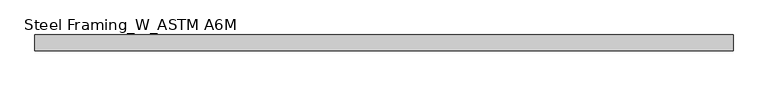
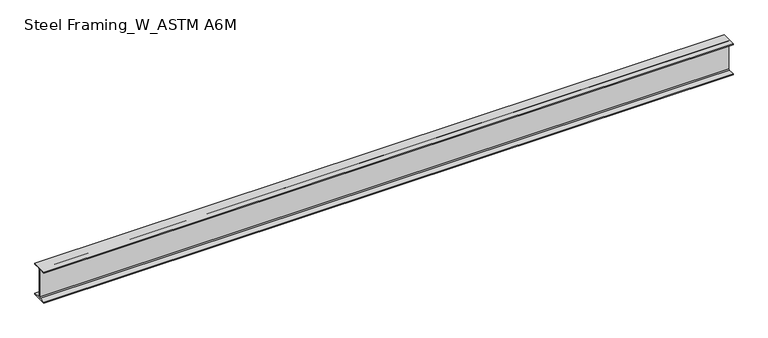
"""IFC4 building model written with IfcOpenShell, lengths in millimetres: beam geometry, Steel Framing_W_ASTM A6M : H_SB_AR_S02_W360x51_G3."""

import ifcopenshell
import ifcopenshell.guid

model = None  # the IFC model being written
_history = None  # IfcOwnerHistory: only IFC2X3 demands one
_inside = {}  # id of a spatial element -> (the spatial element, [elements in it])
_under = {}  # id of a project, library or spatial element -> (it, [spatial elements below it])
_declared = {}  # id of a project -> (the project, [libraries it declares])
_typed = {}  # id of a type object -> (the type object, [elements of that type])
_made_of = {}  # id of a material, layer set ... -> (it, [elements and type objects made of it])


def new_model(schema):
    """Start an empty IFC model of exactly this schema.

    Asked for "IFC4X3", IfcOpenShell would pick the latest addendum, in which some entities
    have other attributes; the version numbers below select the first issue.
    IFC2X3 requires an IfcOwnerHistory on every rooted entity: one is made here for all.
    """
    global model, _history
    if schema == "IFC4X3":
        model = ifcopenshell.file(schema_version=(4, 3, 0, 0))
    else:
        model = ifcopenshell.file(schema=schema)
    _inside.clear()
    _under.clear()
    _declared.clear()
    _typed.clear()
    _made_of.clear()
    _history = None
    if model.schema == "IFC2X3":
        org = make("IfcOrganization", Name="unknown")
        user = make(
            "IfcPersonAndOrganization",
            ThePerson=make("IfcPerson", FamilyName="unknown"),
            TheOrganization=org,
        )
        app = make(
            "IfcApplication",
            ApplicationDeveloper=org,
            Version="unknown",
            ApplicationFullName="unknown",
            ApplicationIdentifier="unknown",
        )
        _history = make(
            "IfcOwnerHistory",
            OwningUser=user,
            OwningApplication=app,
            ChangeAction="ADDED",
            CreationDate=0,
        )
    return model


def make(cls, **values):
    """One entity of the class cls with the attributes given. An attribute that is None is left unset."""
    return model.create_entity(
        cls, **{name: value for name, value in values.items() if value is not None}
    )


def rooted(cls, **values):
    """An entity with a GlobalId (a new one), such as an element, a storey or a relation."""
    return make(cls, GlobalId=ifcopenshell.guid.new(), OwnerHistory=_history, **values)


def si_unit(unit_type, name, prefix=None):
    """IfcSIUnit, for example si_unit("LENGTHUNIT", "METRE", prefix="MILLI")."""
    return make("IfcSIUnit", UnitType=unit_type, Prefix=prefix, Name=name)


def assignment(units):
    """IfcUnitAssignment: the units of a project."""
    return None if units is None else make("IfcUnitAssignment", Units=units)


def point(xyz):
    """IfcCartesianPoint."""
    return None if xyz is None else make("IfcCartesianPoint", Coordinates=xyz)


def direction(xyz):
    """IfcDirection."""
    return None if xyz is None else make("IfcDirection", DirectionRatios=xyz)


def frame(location, z_axis=None, x_axis=None):
    """IfcAxis2Placement3D, a coordinate frame: its origin and axes. An axis left out is left unset."""
    return make(
        "IfcAxis2Placement3D",
        Location=point(location),
        Axis=direction(z_axis),
        RefDirection=direction(x_axis),
    )


def frame_2d(location, x_axis=None):
    """IfcAxis2Placement2D, a coordinate frame in the plane: its origin and x axis."""
    return make(
        "IfcAxis2Placement2D", Location=point(location), RefDirection=direction(x_axis)
    )


def origin():
    """The frame at (0, 0, 0) with its axes left unset."""
    return frame((0.0, 0.0, 0.0))


def place(relative_to, where):
    """IfcLocalPlacement: puts the frame where relative to a parent placement (None: the world)."""
    return make(
        "IfcLocalPlacement", PlacementRelTo=relative_to, RelativePlacement=where
    )


def context(
    kind, dimensions, precision=None, world=None, true_north=None, identifier=None
):
    """IfcGeometricRepresentationContext, for example the 3D "Model" context."""
    return make(
        "IfcGeometricRepresentationContext",
        ContextIdentifier=identifier,
        ContextType=kind,
        CoordinateSpaceDimension=dimensions,
        Precision=precision,
        WorldCoordinateSystem=world,
        TrueNorth=true_north,
    )


def project(units=None, contexts=None):
    """IfcProject with its units and contexts."""
    return rooted(
        "IfcProject",
        Name="project",
        RepresentationContexts=contexts,
        UnitsInContext=assignment(units),
    )


def spatial(cls, under=None, at=None, **own):
    """A site, building, storey or space (cls), placed at a placement, below another one or the project."""
    s = rooted(cls, ObjectPlacement=at, **own)
    if under is not None:
        _under.setdefault(under.id(), (under, []))[1].append(s)
    return s


def polyline(points):
    """IfcPolyline through the points."""
    return make("IfcPolyline", Points=[point(p) for p in points])


def circle_curve(where, radius):
    """IfcCircle in the frame where."""
    return make("IfcCircle", Position=where, Radius=radius)


def trimmed(basis, trim1, trim2, sense, master):
    """IfcTrimmedCurve: the piece of a basis curve between two trims."""
    return make(
        "IfcTrimmedCurve",
        BasisCurve=basis,
        Trim1=trim1,
        Trim2=trim2,
        SenseAgreement=sense,
        MasterRepresentation=master,
    )


def segment(curve, same_sense, transition):
    """IfcCompositeCurveSegment."""
    return make(
        "IfcCompositeCurveSegment",
        Transition=transition,
        SameSense=same_sense,
        ParentCurve=curve,
    )


def composite_curve(segments, self_intersect=None):
    """IfcCompositeCurve: segments joined end to end."""
    return make("IfcCompositeCurve", Segments=segments, SelfIntersect=self_intersect)


def outline(outer, holes=None, kind="AREA"):
    """IfcArbitraryClosedProfileDef: a profile drawn as a closed curve; with holes, ...WithVoids."""
    if holes is None:
        return make("IfcArbitraryClosedProfileDef", ProfileType=kind, OuterCurve=outer)
    return make(
        "IfcArbitraryProfileDefWithVoids",
        ProfileType=kind,
        OuterCurve=outer,
        InnerCurves=holes,
    )


def extrude(swept, where, along, depth):
    """IfcExtrudedAreaSolid: the profile swept, set in the frame where, extruded along a direction by depth."""
    return make(
        "IfcExtrudedAreaSolid",
        SweptArea=swept,
        Position=where,
        ExtrudedDirection=direction(along),
        Depth=depth,
    )


def shape(context_of_items, identifier, shape_type, items):
    """IfcShapeRepresentation: the items that make up one representation, for example the "Body"."""
    return make(
        "IfcShapeRepresentation",
        ContextOfItems=context_of_items,
        RepresentationIdentifier=identifier,
        RepresentationType=shape_type,
        Items=items,
    )


def source(mapping_origin, context_of_items, identifier, shape_type, items):
    """IfcRepresentationMap: a shape defined once, which mapped items show again and again."""
    return make(
        "IfcRepresentationMap",
        MappingOrigin=mapping_origin,
        MappedRepresentation=shape(context_of_items, identifier, shape_type, items),
    )


def transform(
    local_origin,
    x_axis=None,
    y_axis=None,
    z_axis=None,
    scale=None,
    scale2=None,
    scale3=None,
    uniform=True,
):
    """IfcCartesianTransformationOperator3D, or its non-uniform kind. x_axis, y_axis, z_axis: its Axis1, 2, 3."""
    if uniform:
        return make(
            "IfcCartesianTransformationOperator3D",
            Axis1=direction(x_axis),
            Axis2=direction(y_axis),
            LocalOrigin=point(local_origin),
            Scale=scale,
            Axis3=direction(z_axis),
        )
    return make(
        "IfcCartesianTransformationOperator3DnonUniform",
        Axis1=direction(x_axis),
        Axis2=direction(y_axis),
        LocalOrigin=point(local_origin),
        Scale=scale,
        Axis3=direction(z_axis),
        Scale2=scale2,
        Scale3=scale3,
    )


def mapped(mapping_source, mapping_target):
    """IfcMappedItem: shows the shape of a source again, moved by a transform."""
    return make(
        "IfcMappedItem", MappingSource=mapping_source, MappingTarget=mapping_target
    )


def made_of(thing, what):
    """Note that an element or type object is made of a material, layer set ...; save() writes the relation."""
    if what is not None:
        _made_of.setdefault(what.id(), (what, []))[1].append(thing)
    return thing


def element(
    cls,
    number,
    at=None,
    inside=None,
    cuts=None,
    type_object=None,
    material=None,
    context=None,
    identifier="Body",
    shape_type=None,
    held_by="IfcProductDefinitionShape",
    body=None,
    shapes=None,
    **own,
):
    """One element of the class cls, such as IfcWall. Its Tag is "e" and its number.

    at: its placement. inside: the storey or other place that contains it. cuts: it is an
    opening in that element (IfcRelVoidsElement). A single representation is given by context,
    identifier, shape_type and body (its items); several are given by shapes. held_by: the class
    of the entity that holds the representations. save() writes the other relations.
    """
    e = rooted(cls, Tag="e%d" % number, ObjectPlacement=at, **own)
    if body is not None:
        shapes = [shape(context, identifier, shape_type, body)]
    if shapes is not None:
        e.Representation = make(held_by, Representations=shapes)
    if inside is not None:
        _inside.setdefault(inside.id(), (inside, []))[1].append(e)
    if cuts is not None:
        rooted(
            "IfcRelVoidsElement", RelatingBuildingElement=cuts, RelatedOpeningElement=e
        )
    if type_object is not None:
        _typed.setdefault(type_object.id(), (type_object, []))[1].append(e)
    return made_of(e, material)


def aggregate(whole, parts):
    """IfcRelAggregates: a whole, such as a stair, and the parts it consists of."""
    return rooted("IfcRelAggregates", RelatingObject=whole, RelatedObjects=parts)


def save(model, path):
    """Write the relations noted so far, then the file.

    IfcRelAggregates (storeys below a building ...), IfcRelContainedInSpatialStructure (elements
    in a storey), IfcRelDefinesByType, IfcRelAssociatesMaterial and IfcRelDeclares: one each for
    every whole, place, type object, material and project.
    """
    for whole, parts in _under.values():
        aggregate(whole, parts)
    for where, things in _inside.values():
        rooted(
            "IfcRelContainedInSpatialStructure",
            RelatedElements=things,
            RelatingStructure=where,
        )
    for kind, things in _typed.values():
        rooted("IfcRelDefinesByType", RelatedObjects=things, RelatingType=kind)
    for what, things in _made_of.values():
        rooted("IfcRelAssociatesMaterial", RelatedObjects=things, RelatingMaterial=what)
    for by, libraries in _declared.values():
        rooted("IfcRelDeclares", RelatingContext=by, RelatedDefinitions=libraries)
    model.write(path)


def steel_framing_w_astm_a6m_5f06bcad(model_context):
    return source(origin(), model_context, "Body", "SweptSolid", [
        extrude(outline(composite_curve([segment(polyline([(85.5, -166.4), (85.5, -178.0), (-85.5, -178.0), (-85.5, -166.4), (-13.72, -166.4)]), True, "CONTINUOUS"), segment(trimmed(circle_curve(frame_2d((-13.72, -156.3)), 10.1), [point((-13.72, -166.4))], [point((-3.62, -156.3))], True, "CARTESIAN"), True, "CONTINUOUS"), segment(polyline([(-3.62, -156.3), (-3.62, 156.3)]), True, "CONTINUOUS"), segment(trimmed(circle_curve(frame_2d((-13.72, 156.3)), 10.1), [point((-3.62, 156.3))], [point((-13.72, 166.4))], True, "CARTESIAN"), True, "CONTINUOUS"), segment(polyline([(-13.72, 166.4), (-85.5, 166.4), (-85.5, 178.0), (85.5, 178.0), (85.5, 166.4), (13.72, 166.4)]), True, "CONTINUOUS"), segment(trimmed(circle_curve(frame_2d((13.72, 156.3)), 10.1), [point((13.72, 166.4))], [point((3.62, 156.3))], True, "CARTESIAN"), True, "CONTINUOUS"), segment(polyline([(3.62, 156.3), (3.62, -156.3)]), True, "CONTINUOUS"), segment(trimmed(circle_curve(frame_2d((13.72, -156.3)), 10.1), [point((3.62, -156.3))], [point((13.72, -166.4))], True, "CARTESIAN"), True, "CONTINUOUS"), segment(polyline([(13.72, -166.4), (85.5, -166.4)]), True, "CONTINUOUS")], self_intersect=False)), frame((-3753.8, 0.0, 0.0), z_axis=(1.0, 0.0, 0.0), x_axis=(0.0, 1.0, 0.0)), (0.0, 0.0, 1.0), 7507.6),
    ])


if __name__ == "__main__":
    model = new_model("IFC4")
    model_context = context("Model", 3, world=origin())
    ifc_project = project(units=[si_unit("LENGTHUNIT", "METRE", prefix="MILLI")], contexts=[model_context])
    site = spatial("IfcSite", under=ifc_project)
    building = spatial("IfcBuilding", under=site)
    placement = place(None, origin())
    steel_framing_w_astm_a6m_shape = steel_framing_w_astm_a6m_5f06bcad(model_context)
    element("IfcBeam", 1, ObjectType="Steel Framing_W_ASTM A6M : H_SB_AR_S02_W360x51_G3", at=placement, inside=building, context=model_context, shape_type="MappedRepresentation", body=[
        mapped(steel_framing_w_astm_a6m_shape, transform((0.0, 0.0, 0.0), x_axis=(1.0, 0.0, 0.0), y_axis=(0.0, 1.0, 0.0), z_axis=(0.0, 0.0, 1.0))),
    ])
    save(model, "model.ifc")

# Revit data of these elements
# Type "Steel Framing_W_ASTM A6M : H_SB_AR_S02_W360x51_G3"
#   Type Mark = "G3"
#   Section Name Key = "W14x34"
#   Width = 17.1 cm
#   Web Thickness = 0.724 cm
#   Web Fillet = 1.01 cm
#   Warping Constant = 287000.0 cm⁶
#   Torsional Moment of Inertia = 23.70 cm⁴
#   Section Area = 64.5 cm²
#   Plastic Modulus weak axis = 174.0 cm³
#   Plastic Modulus strong axis = 895.0 cm³
#   Perimeter = 1.36 m²/m
#   Nominal Weight = 51.00 kgf/m
#   Moment of Inertia weak axis = 970.00 cm⁴
#   Moment of Inertia strong axis = 14200.00 cm⁴
#   Height = 35.6 cm
#   Flange Thickness = 1.16 cm
#   Elastic Modulus weak axis = 113.0 cm³
#   Elastic Modulus strong axis = 796.0 cm³
#   Centroid Vertical = 17.8 cm
#   Centroid Horizontal = 8.55 cm
#   Length [instance default] = 1500 mm
#   Structural Material [instance default] = Steel, 45-345
#   Bolt Spacing = 0
#   Assembly Code = ""
# Element 1 (IfcBeam, "Steel Framing_W_ASTM A6M : H_SB_AR_S02_W360x51_G3")
#   Materials on its faces: "Steel, 45-345"
# Materials
#   "Steel, 45-345": class "Metal", colour RGB 189 187 185, transparency 0, Description = "Steel 345 MPa", Cost = 0
